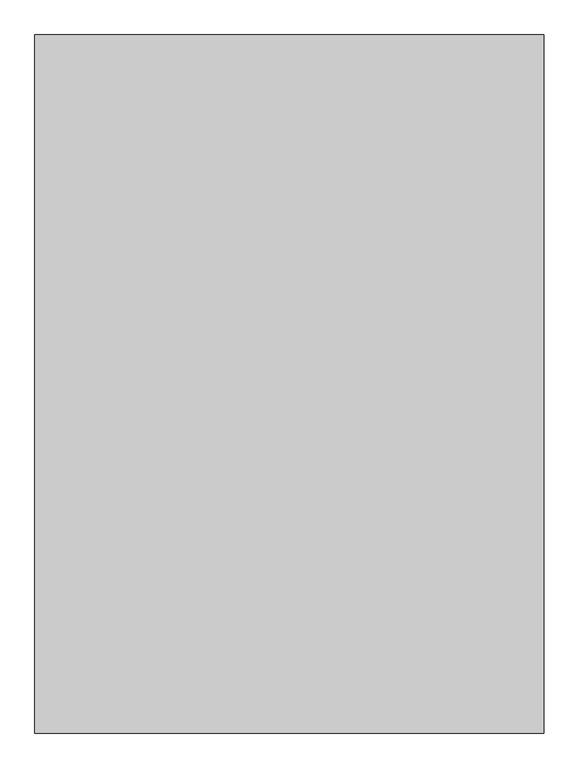
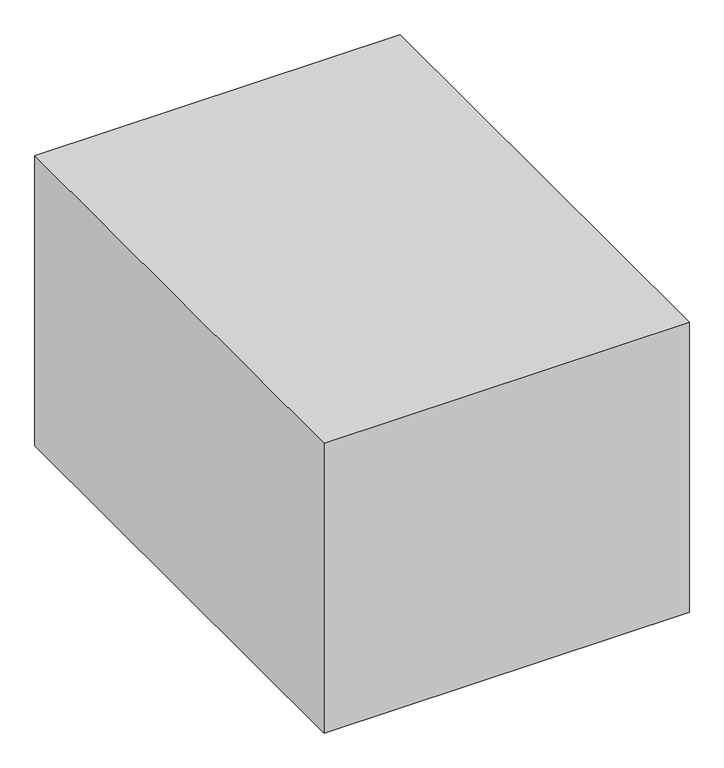
"""IFC4 building model written with IfcOpenShell, lengths in millimetres: proxy geometry, Space Planning Box_hec : Space Planning Box_hec."""

from ifc_helpers import new_model, si_unit, origin, origin_with_axes, place, context, project, spatial, polyline, outline, extrude, source, transform, mapped, element, save


def generic_models_228d8ca4(model_context):
    return source(origin(), model_context, "Body", "SweptSolid", [
        extrude(outline(polyline([(3100.0, 4250.0), (3100.0, -4250.0), (-3100.0, -4250.0), (-3100.0, 4250.0), (3100.0, 4250.0)])), origin_with_axes(), (0.0, 0.0, 1.0), 5200.0),
    ])


if __name__ == "__main__":
    model = new_model("IFC4")
    model_context = context("Model", 3, world=origin())
    ifc_project = project(units=[si_unit("LENGTHUNIT", "METRE", prefix="MILLI")], contexts=[model_context])
    site = spatial("IfcSite", under=ifc_project)
    building = spatial("IfcBuilding", under=site)
    placement = place(None, origin())
    generic_models_shape = generic_models_228d8ca4(model_context)
    element("IfcBuildingElementProxy", 1, Name="Space Planning Box_hec : Space Planning Box_hec", ObjectType="Space Planning Box_hec : Space Planning Box_hec", at=placement, inside=building, context=model_context, shape_type="MappedRepresentation", body=[
        mapped(generic_models_shape, transform((0.0, 0.0, 0.0), x_axis=(1.0, 0.0, 0.0), y_axis=(0.0, 1.0, 0.0), z_axis=(0.0, 0.0, 1.0))),
    ])
    save(model, "model.ifc")

# Revit data of these elements
# Type "Space Planning Box_hec : Space Planning Box_hec"
#   Type Comments = "..."
#   Room Name [instance default] = "?"
#   Interior Finish [instance default] = ""
#   Exterior Finish [instance default] = ""
#   Department [instance default] = ""
#   Assembly Code = "..."
#   ceiling height [instance default] = 0
#   Width [instance default] = 1524 mm
#   Program Area [instance default] = 0.00 m²
#   Length [instance default] = 1524 mm
#   Height [instance default] = 1524 mm
#   Area [instance default] = 2.32258 m²
#   Fill Color [instance default] = Cyan
#   Default Elevation = 0
# Element 1 (IfcBuildingElementProxy, "Space Planning Box_hec : Space Planning Box_hec")
#   Room Name = "Meeting Room-1"
#   Interior Finish = "IW1..N/A,,WB2..N/A,,FL6..N/A,,CL4..N/A"
#   Exterior Finish = "RF1..N/A,,EW1..N/A"
#   Department = "AR"
#   ceiling height = 2700
#   Width = 6200 mm
#   Program Area = 52.70 m²
#   Length = 8500 mm
#   Height = 5200 mm
#   Area = 52.70 m²
#   Materials on its faces: "Cyan"
# Materials
#   "Cyan": class "Generic", colour RGB 0 255 255, transparency 0.2, Cost = 0
